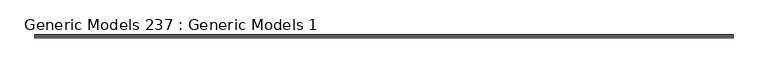
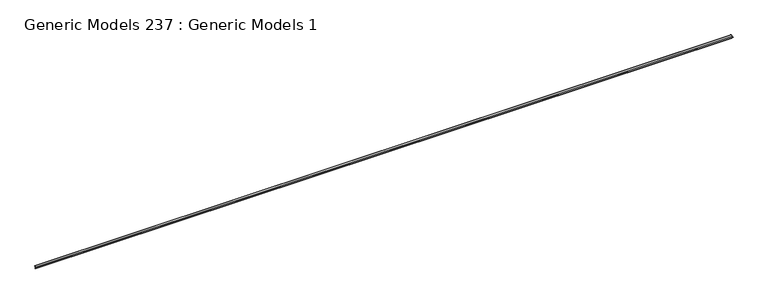
"""IFC4 building model written with IfcOpenShell, lengths in millimetres: proxy geometry, Generic Models 237 : Generic Models 1."""

from ifc_helpers import new_model, si_unit, point, frame, frame_2d, origin, place, context, project, spatial, polyline, circle_curve, trimmed, segment, composite_curve, outline, extrude, source, transform, mapped, element, save


def generic_models_237_generic_models_1_e36d9882(model_context):
    return source(origin(), model_context, "Body", "SweptSolid", [
        extrude(outline(composite_curve([segment(trimmed(circle_curve(frame_2d((-29147.3678344, 127165.3167873)), 1.4342127), [point((-29148.0229895, 127166.5926156))], [point((-29146.0920061, 127164.6616323))], False, "CARTESIAN"), True, "CONTINUOUS"), segment(polyline([(-29146.0920061, 127164.6616323), (-29165.6186218, 127126.6361176), (-29165.6186218, 127088.5361176), (-29166.8886218, 127088.5361176), (-29166.8886218, 127126.9431414), (-29146.9883821, 127165.6962396), (-29185.7414804, 127145.796), (-29224.1485041, 127145.796), (-29224.1485041, 127147.066), (-29186.0485041, 127147.066), (-29148.0229895, 127166.5926156)]), True, "CONTINUOUS")], self_intersect=False)), frame((-20998.9733045, 0.0, 0.0), z_axis=(1.0, 0.0, 0.0), x_axis=(0.0, 1.0, 0.0)), (0.0, 0.0, 1.0), 19050.0),
    ])


if __name__ == "__main__":
    model = new_model("IFC4")
    model_context = context("Model", 3, world=origin())
    ifc_project = project(units=[si_unit("LENGTHUNIT", "METRE", prefix="MILLI")], contexts=[model_context])
    site = spatial("IfcSite", under=ifc_project)
    building = spatial("IfcBuilding", under=site)
    placement = place(None, origin())
    generic_models_237_generic_models_1_shape = generic_models_237_generic_models_1_e36d9882(model_context)
    element("IfcBuildingElementProxy", 1, Name="Generic Models 237 : Generic Models 1", ObjectType="Generic Models 237 : Generic Models 1", at=placement, inside=building, context=model_context, shape_type="MappedRepresentation", body=[
        mapped(generic_models_237_generic_models_1_shape, transform((0.0, 0.0, 0.0), x_axis=(1.0, 0.0, 0.0), y_axis=(0.0, 1.0, 0.0), z_axis=(0.0, 0.0, 1.0))),
    ])
    save(model, "model.ifc")

# Revit data of these elements
# Element 1 (IfcBuildingElementProxy, "Generic Models 237 : Generic Models 1")
#   Materials on its faces: "_CONTINIOUS 16 GA. COPPER CORNER BEAD"
# Materials
#   "_CONTINIOUS 16 GA. COPPER CORNER BEAD": class "Generic", colour RGB 253 192 103, transparency 0, Cost = 0
